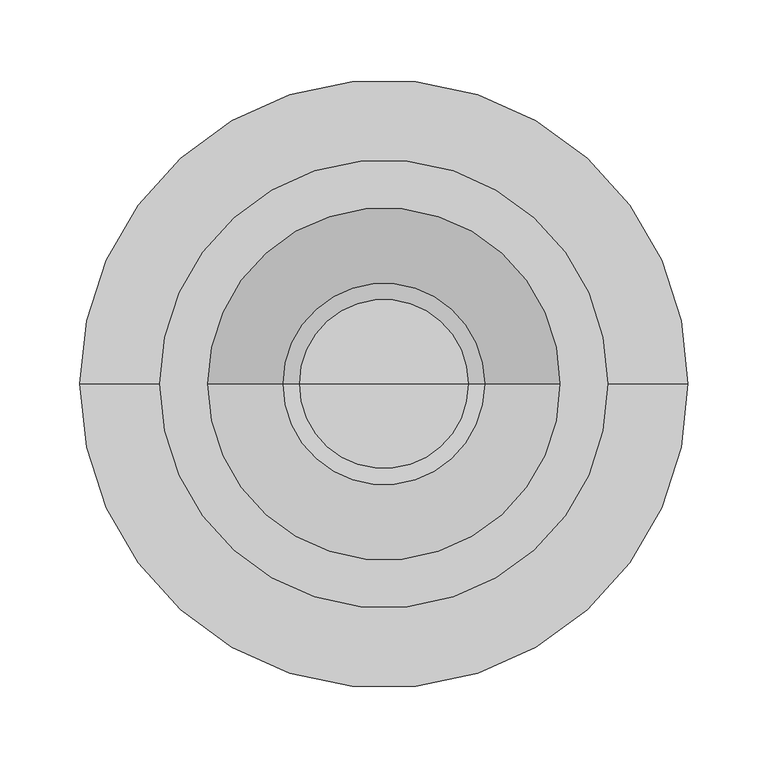
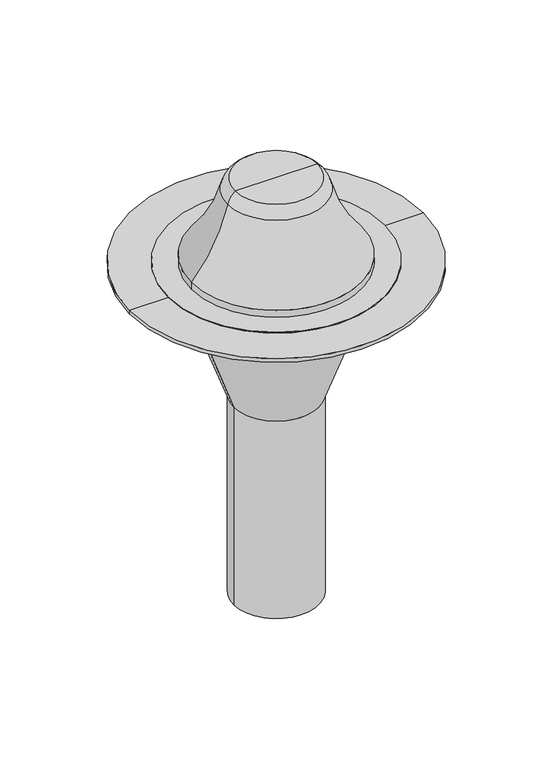
"""IFC4 building model written with IfcOpenShell, lengths in millimetres: proxy geometry, TN_Воронка с обжимным фланцем : Воронка с обжимным закручивающемся фланцем без обогрева Ø110х450мм."""

import ifcopenshell
import ifcopenshell.guid

model = None  # the IFC model being written
_history = None  # IfcOwnerHistory: only IFC2X3 demands one
_inside = {}  # id of a spatial element -> (the spatial element, [elements in it])
_under = {}  # id of a project, library or spatial element -> (it, [spatial elements below it])
_declared = {}  # id of a project -> (the project, [libraries it declares])
_typed = {}  # id of a type object -> (the type object, [elements of that type])
_made_of = {}  # id of a material, layer set ... -> (it, [elements and type objects made of it])


def new_model(schema):
    """Start an empty IFC model of exactly this schema.

    Asked for "IFC4X3", IfcOpenShell would pick the latest addendum, in which some entities
    have other attributes; the version numbers below select the first issue.
    IFC2X3 requires an IfcOwnerHistory on every rooted entity: one is made here for all.
    """
    global model, _history
    if schema == "IFC4X3":
        model = ifcopenshell.file(schema_version=(4, 3, 0, 0))
    else:
        model = ifcopenshell.file(schema=schema)
    _inside.clear()
    _under.clear()
    _declared.clear()
    _typed.clear()
    _made_of.clear()
    _history = None
    if model.schema == "IFC2X3":
        org = make("IfcOrganization", Name="unknown")
        user = make(
            "IfcPersonAndOrganization",
            ThePerson=make("IfcPerson", FamilyName="unknown"),
            TheOrganization=org,
        )
        app = make(
            "IfcApplication",
            ApplicationDeveloper=org,
            Version="unknown",
            ApplicationFullName="unknown",
            ApplicationIdentifier="unknown",
        )
        _history = make(
            "IfcOwnerHistory",
            OwningUser=user,
            OwningApplication=app,
            ChangeAction="ADDED",
            CreationDate=0,
        )
    return model


def make(cls, **values):
    """One entity of the class cls with the attributes given. An attribute that is None is left unset."""
    return model.create_entity(
        cls, **{name: value for name, value in values.items() if value is not None}
    )


def rooted(cls, **values):
    """An entity with a GlobalId (a new one), such as an element, a storey or a relation."""
    return make(cls, GlobalId=ifcopenshell.guid.new(), OwnerHistory=_history, **values)


def si_unit(unit_type, name, prefix=None):
    """IfcSIUnit, for example si_unit("LENGTHUNIT", "METRE", prefix="MILLI")."""
    return make("IfcSIUnit", UnitType=unit_type, Prefix=prefix, Name=name)


def assignment(units):
    """IfcUnitAssignment: the units of a project."""
    return None if units is None else make("IfcUnitAssignment", Units=units)


def point(xyz):
    """IfcCartesianPoint."""
    return None if xyz is None else make("IfcCartesianPoint", Coordinates=xyz)


def direction(xyz):
    """IfcDirection."""
    return None if xyz is None else make("IfcDirection", DirectionRatios=xyz)


def frame(location, z_axis=None, x_axis=None):
    """IfcAxis2Placement3D, a coordinate frame: its origin and axes. An axis left out is left unset."""
    return make(
        "IfcAxis2Placement3D",
        Location=point(location),
        Axis=direction(z_axis),
        RefDirection=direction(x_axis),
    )


def frame_2d(location, x_axis=None):
    """IfcAxis2Placement2D, a coordinate frame in the plane: its origin and x axis."""
    return make(
        "IfcAxis2Placement2D", Location=point(location), RefDirection=direction(x_axis)
    )


def origin():
    """The frame at (0, 0, 0) with its axes left unset."""
    return frame((0.0, 0.0, 0.0))


def origin_with_axes():
    """The frame at (0, 0, 0) with the z axis (0, 0, 1) and the x axis (1, 0, 0) written out."""
    return frame((0.0, 0.0, 0.0), z_axis=(0.0, 0.0, 1.0), x_axis=(1.0, 0.0, 0.0))


def origin_2d():
    """The frame at (0, 0) in the plane with its x axis left unset."""
    return frame_2d((0.0, 0.0))


def place(relative_to, where):
    """IfcLocalPlacement: puts the frame where relative to a parent placement (None: the world)."""
    return make(
        "IfcLocalPlacement", PlacementRelTo=relative_to, RelativePlacement=where
    )


def context(
    kind, dimensions, precision=None, world=None, true_north=None, identifier=None
):
    """IfcGeometricRepresentationContext, for example the 3D "Model" context."""
    return make(
        "IfcGeometricRepresentationContext",
        ContextIdentifier=identifier,
        ContextType=kind,
        CoordinateSpaceDimension=dimensions,
        Precision=precision,
        WorldCoordinateSystem=world,
        TrueNorth=true_north,
    )


def project(units=None, contexts=None):
    """IfcProject with its units and contexts."""
    return rooted(
        "IfcProject",
        Name="project",
        RepresentationContexts=contexts,
        UnitsInContext=assignment(units),
    )


def spatial(cls, under=None, at=None, **own):
    """A site, building, storey or space (cls), placed at a placement, below another one or the project."""
    s = rooted(cls, ObjectPlacement=at, **own)
    if under is not None:
        _under.setdefault(under.id(), (under, []))[1].append(s)
    return s


def polyline(points):
    """IfcPolyline through the points."""
    return make("IfcPolyline", Points=[point(p) for p in points])


def circle_curve(where, radius):
    """IfcCircle in the frame where."""
    return make("IfcCircle", Position=where, Radius=radius)


def ellipse_curve(where, semi_axis1, semi_axis2):
    """IfcEllipse in the frame where."""
    return make(
        "IfcEllipse", Position=where, SemiAxis1=semi_axis1, SemiAxis2=semi_axis2
    )


def trimmed(basis, trim1, trim2, sense, master):
    """IfcTrimmedCurve: the piece of a basis curve between two trims."""
    return make(
        "IfcTrimmedCurve",
        BasisCurve=basis,
        Trim1=trim1,
        Trim2=trim2,
        SenseAgreement=sense,
        MasterRepresentation=master,
    )


def segment(curve, same_sense, transition):
    """IfcCompositeCurveSegment."""
    return make(
        "IfcCompositeCurveSegment",
        Transition=transition,
        SameSense=same_sense,
        ParentCurve=curve,
    )


def composite_curve(segments, self_intersect=None):
    """IfcCompositeCurve: segments joined end to end."""
    return make("IfcCompositeCurve", Segments=segments, SelfIntersect=self_intersect)


def outline(outer, holes=None, kind="AREA"):
    """IfcArbitraryClosedProfileDef: a profile drawn as a closed curve; with holes, ...WithVoids."""
    if holes is None:
        return make("IfcArbitraryClosedProfileDef", ProfileType=kind, OuterCurve=outer)
    return make(
        "IfcArbitraryProfileDefWithVoids",
        ProfileType=kind,
        OuterCurve=outer,
        InnerCurves=holes,
    )


def extrude(swept, where, along, depth):
    """IfcExtrudedAreaSolid: the profile swept, set in the frame where, extruded along a direction by depth."""
    return make(
        "IfcExtrudedAreaSolid",
        SweptArea=swept,
        Position=where,
        ExtrudedDirection=direction(along),
        Depth=depth,
    )


def shape(context_of_items, identifier, shape_type, items):
    """IfcShapeRepresentation: the items that make up one representation, for example the "Body"."""
    return make(
        "IfcShapeRepresentation",
        ContextOfItems=context_of_items,
        RepresentationIdentifier=identifier,
        RepresentationType=shape_type,
        Items=items,
    )


def source(mapping_origin, context_of_items, identifier, shape_type, items):
    """IfcRepresentationMap: a shape defined once, which mapped items show again and again."""
    return make(
        "IfcRepresentationMap",
        MappingOrigin=mapping_origin,
        MappedRepresentation=shape(context_of_items, identifier, shape_type, items),
    )


def transform(
    local_origin,
    x_axis=None,
    y_axis=None,
    z_axis=None,
    scale=None,
    scale2=None,
    scale3=None,
    uniform=True,
):
    """IfcCartesianTransformationOperator3D, or its non-uniform kind. x_axis, y_axis, z_axis: its Axis1, 2, 3."""
    if uniform:
        return make(
            "IfcCartesianTransformationOperator3D",
            Axis1=direction(x_axis),
            Axis2=direction(y_axis),
            LocalOrigin=point(local_origin),
            Scale=scale,
            Axis3=direction(z_axis),
        )
    return make(
        "IfcCartesianTransformationOperator3DnonUniform",
        Axis1=direction(x_axis),
        Axis2=direction(y_axis),
        LocalOrigin=point(local_origin),
        Scale=scale,
        Axis3=direction(z_axis),
        Scale2=scale2,
        Scale3=scale3,
    )


def mapped(mapping_source, mapping_target):
    """IfcMappedItem: shows the shape of a source again, moved by a transform."""
    return make(
        "IfcMappedItem", MappingSource=mapping_source, MappingTarget=mapping_target
    )


def made_of(thing, what):
    """Note that an element or type object is made of a material, layer set ...; save() writes the relation."""
    if what is not None:
        _made_of.setdefault(what.id(), (what, []))[1].append(thing)
    return thing


def element(
    cls,
    number,
    at=None,
    inside=None,
    cuts=None,
    type_object=None,
    material=None,
    context=None,
    identifier="Body",
    shape_type=None,
    held_by="IfcProductDefinitionShape",
    body=None,
    shapes=None,
    **own,
):
    """One element of the class cls, such as IfcWall. Its Tag is "e" and its number.

    at: its placement. inside: the storey or other place that contains it. cuts: it is an
    opening in that element (IfcRelVoidsElement). A single representation is given by context,
    identifier, shape_type and body (its items); several are given by shapes. held_by: the class
    of the entity that holds the representations. save() writes the other relations.
    """
    e = rooted(cls, Tag="e%d" % number, ObjectPlacement=at, **own)
    if body is not None:
        shapes = [shape(context, identifier, shape_type, body)]
    if shapes is not None:
        e.Representation = make(held_by, Representations=shapes)
    if inside is not None:
        _inside.setdefault(inside.id(), (inside, []))[1].append(e)
    if cuts is not None:
        rooted(
            "IfcRelVoidsElement", RelatingBuildingElement=cuts, RelatedOpeningElement=e
        )
    if type_object is not None:
        _typed.setdefault(type_object.id(), (type_object, []))[1].append(e)
    return made_of(e, material)


def aggregate(whole, parts):
    """IfcRelAggregates: a whole, such as a stair, and the parts it consists of."""
    return rooted("IfcRelAggregates", RelatingObject=whole, RelatedObjects=parts)


def save(model, path):
    """Write the relations noted so far, then the file.

    IfcRelAggregates (storeys below a building ...), IfcRelContainedInSpatialStructure (elements
    in a storey), IfcRelDefinesByType, IfcRelAssociatesMaterial and IfcRelDeclares: one each for
    every whole, place, type object, material and project.
    """
    for whole, parts in _under.values():
        aggregate(whole, parts)
    for where, things in _inside.values():
        rooted(
            "IfcRelContainedInSpatialStructure",
            RelatedElements=things,
            RelatingStructure=where,
        )
    for kind, things in _typed.values():
        rooted("IfcRelDefinesByType", RelatedObjects=things, RelatingType=kind)
    for what, things in _made_of.values():
        rooted("IfcRelAssociatesMaterial", RelatedObjects=things, RelatingMaterial=what)
    for by, libraries in _declared.values():
        rooted("IfcRelDeclares", RelatingContext=by, RelatedDefinitions=libraries)
    model.write(path)


def plane_surface(at):
    """IfcPlane: the flat surface through the origin of the frame at, square to its z axis."""
    return make("IfcPlane", Position=at)


def cylinder_surface(at, radius):
    """IfcCylindricalSurface: all points at the distance radius from the z axis of the frame at."""
    return make("IfcCylindricalSurface", Position=at, Radius=radius)


def revolved_surface(curve, axis_point, axis_direction):
    """IfcSurfaceOfRevolution: the curve turned about the line through axis_point along axis_direction."""
    return make(
        "IfcSurfaceOfRevolution",
        SweptCurve=make("IfcArbitraryOpenProfileDef", ProfileType="CURVE", Curve=curve),
        AxisPosition=make("IfcAxis1Placement", Location=point(axis_point), Axis=direction(axis_direction)),
    )


def advanced_brep(points, edges, surfaces, faces):
    """IfcAdvancedBrep: a solid bounded by faces that lie on surfaces and meet in shared edges.

    An edge is (start, end): straight between two places in points (the first is 0);
    or (start, end, curve); or (start, end, curve, False) where it runs against its curve.
    A face is (place in surfaces, loops), or (place, loops, False) where it looks against
    its surface's normal. A loop lists edges by number (the first is 1), with a minus sign
    where the edge is run from its end to its start. The first loop is the outer one.
    """
    corners = [point(p) for p in points]
    vertices = [make("IfcVertexPoint", VertexGeometry=c) for c in corners]
    made = []
    for start, end, *more in edges:
        made.append(
            make(
                "IfcEdgeCurve",
                EdgeStart=vertices[start],
                EdgeEnd=vertices[end],
                EdgeGeometry=more[0] if more else make("IfcPolyline", Points=[corners[start], corners[end]]),
                SameSense=more[1] if len(more) > 1 else True,
            )
        )
    hull = []
    for where, loops, *sense in faces:
        bounds = []
        for j, loop in enumerate(loops):
            ring = [make("IfcOrientedEdge", EdgeElement=made[abs(k) - 1], Orientation=k > 0) for k in loop]
            bounds.append(
                make(
                    "IfcFaceOuterBound" if j == 0 else "IfcFaceBound",
                    Bound=make("IfcEdgeLoop", EdgeList=ring),
                    Orientation=True,
                )
            )
        hull.append(make("IfcAdvancedFace", Bounds=bounds, FaceSurface=surfaces[where], SameSense=sense[0] if sense else True))
    return make("IfcAdvancedBrep", Outer=make("IfcClosedShell", CfsFaces=hull))


def specialty_equipment_201b4a6f(model_context):
    return source(origin(), model_context, "Body", "SolidModel", [
        advanced_brep(
        [(110.0556416, 0.0, 0.0), (-110.0556416, 0.0, 0.0), (-110.0556416, 0.0, 10.0), (110.0556416, 0.0, 10.0), (0.0, 0.0, 0.0), (52.7728393, 0.0, 115.0), (-52.7728393, 0.0, 115.0), (0.0, 0.0, 115.0), (62.9807579, 0.0, 100.6532382), (-62.9807579, 0.0, 100.6532382)],
        [
            (0, 1, circle_curve(frame((0.0, 0.0, 0.0), z_axis=(0.0, 0.0, 1.0), x_axis=(-1.0, 0.0, 0.0)), 110.0556416)),
            (1, 2),
            (2, 3, circle_curve(frame((0.0, 0.0, 10.0), z_axis=(0.0, 0.0, -1.0), x_axis=(-1.0, 0.0, 0.0)), 110.0556416)),
            (3, 0),
            (1, 0, circle_curve(frame((0.0, 0.0, 0.0), z_axis=(0.0, 0.0, 1.0), x_axis=(-1.0, 0.0, 0.0)), 110.0556416)),
            (3, 2, circle_curve(frame((0.0, 0.0, 10.0), z_axis=(0.0, 0.0, -1.0), x_axis=(-1.0, 0.0, 0.0)), 110.0556416)),
            (4, 1),
            (0, 4),
            (5, 6, circle_curve(frame((0.0, 0.0, 115.0), z_axis=(0.0, 0.0, 1.0), x_axis=(-1.0, 0.0, 0.0)), 52.7728393)),
            (6, 7),
            (7, 5),
            (6, 5, circle_curve(frame((0.0, 0.0, 115.0), z_axis=(0.0, 0.0, 1.0), x_axis=(-1.0, 0.0, 0.0)), 52.7728393)),
            (8, 9, circle_curve(frame((0.0, 0.0, 100.6532382), z_axis=(0.0, 0.0, 1.0), x_axis=(-1.0, 0.0, 0.0)), 62.9807579)),
            (9, 6, circle_curve(frame((-39.8885443, 0.0, 95.0277285), z_axis=(0.0, 1.0, 0.0), x_axis=(1.0, 0.0, 0.0)), 23.7675553)),
            (5, 8, circle_curve(frame((39.8885443, 0.0, 95.0277285), z_axis=(0.0, 1.0, 0.0), x_axis=(-1.0, 0.0, 0.0)), 23.7675553)),
            (9, 8, circle_curve(frame((0.0, 0.0, 100.6532382), z_axis=(0.0, 0.0, 1.0), x_axis=(-1.0, 0.0, 0.0)), 62.9807579)),
            (2, 9, circle_curve(frame((-271.7387744, 0.0, 151.5089197), z_axis=(0.0, -1.0, 0.0), x_axis=(1.0, 0.0, 0.0)), 214.8632351)),
            (8, 3, circle_curve(frame((271.7387744, 0.0, 151.5089197), z_axis=(0.0, -1.0, 0.0), x_axis=(-1.0, 0.0, 0.0)), 214.8632351)),
        ],
        [
            cylinder_surface(frame((0.0, 0.0, 0.0), z_axis=(0.0, 0.0, -1.0), x_axis=(-1.0, 0.0, 0.0)), 110.0556416),
            plane_surface(frame((0.0, 0.0, 0.0), z_axis=(0.0, 0.0, -1.0), x_axis=(-1.0, 0.0, 0.0))),
            plane_surface(frame((0.0, 0.0, 115.0), z_axis=(0.0, 0.0, 1.0), x_axis=(-1.0, 0.0, 0.0))),
            revolved_surface(trimmed(ellipse_curve(frame((-39.8885443, 0.0, 95.0277285), z_axis=(0.0, -1.0, 0.0), x_axis=(1.0, 0.0, 0.0)), 23.7675553, 23.7675553), [point((-52.7728393, 0.0, 115.0))], [point((-62.9807579, 0.0, 100.6532382))], True, "CARTESIAN"), (0.0, 0.0, 0.0), (0.0, 0.0, -1.0)),
            revolved_surface(trimmed(ellipse_curve(frame((-271.7387744, 0.0, 151.5089197), z_axis=(0.0, 1.0, 0.0), x_axis=(1.0, 0.0, 0.0)), 214.8632351, 214.8632351), [point((-62.9807579, 0.0, 100.6532382))], [point((-110.0556416, 0.0, 10.0))], True, "CARTESIAN"), (0.0, 0.0, 0.0), (0.0, 0.0, -1.0)),
        ],
        [
            (0, [[1, 2, 3, 4]]),
            (0, [[5, -4, 6, -2]]),
            (1, [[7, -1, 8]]),
            (1, [[-8, -5, -7]]),
            (2, [[9, 10, 11]]),
            (2, [[12, -11, -10]]),
            (3, [[13, 14, -9, 15]]),
            (3, [[16, -15, -12, -14]]),
            (4, [[-3, 17, -13, 18]]),
            (4, [[-6, -18, -16, -17]]),
        ],
    ),
        extrude(outline(composite_curve([segment(trimmed(circle_curve(origin_2d(), 140.0), [point((-140.0, 0.0))], [point((140.0, 0.0))], False, "CARTESIAN"), True, "CONTINUOUS"), segment(trimmed(circle_curve(origin_2d(), 140.0), [point((140.0, 0.0))], [point((-140.0, 0.0))], False, "CARTESIAN"), True, "CONTINUOUS")], self_intersect=False), holes=[composite_curve([segment(trimmed(circle_curve(origin_2d(), 110.0556416), [point((-110.0556416, 0.0))], [point((110.0556416, 0.0))], True, "CARTESIAN"), True, "CONTINUOUS"), segment(trimmed(circle_curve(origin_2d(), 110.0556416), [point((110.0556416, 0.0))], [point((-110.0556416, 0.0))], True, "CARTESIAN"), True, "CONTINUOUS")], self_intersect=False)]), origin_with_axes(), (0.0, 0.0, 1.0), 1.0),
        advanced_brep(
        [(0.0, 0.0, -450.0), (-55.0, 0.0, -450.0), (55.0, 0.0, -450.0), (190.0, 0.0, 0.0), (-190.0, 0.0, 0.0), (-83.890873, 0.0, 0.0), (83.890873, 0.0, 0.0), (190.0, 0.0, -5.0), (-190.0, 0.0, -5.0), (93.890873, 0.0, -5.0), (-93.890873, 0.0, -5.0), (55.0, 0.0, -179.9935725), (-55.0, 0.0, -179.9935725), (-93.890873, 0.0, -71.109127), (93.890873, 0.0, -71.109127), (81.9669914, 0.0, -74.7632135), (-81.9669914, 0.0, -74.7632135), (0.0, 0.0, -74.7632135), (83.890873, 0.0, -69.3768397), (-83.890873, 0.0, -69.3768397)],
        [
            (0, 1),
            (1, 2, circle_curve(frame((0.0, 0.0, -450.0), z_axis=(0.0, 0.0, -1.0), x_axis=(-1.0, 0.0, 0.0)), 55.0)),
            (2, 0),
            (2, 1, circle_curve(frame((0.0, 0.0, -450.0), z_axis=(0.0, 0.0, -1.0), x_axis=(-1.0, 0.0, 0.0)), 55.0)),
            (3, 4, circle_curve(frame((0.0, 0.0, 0.0), z_axis=(0.0, 0.0, 1.0), x_axis=(-1.0, 0.0, 0.0)), 190.0)),
            (4, 5),
            (5, 6, circle_curve(frame((0.0, 0.0, 0.0), z_axis=(0.0, 0.0, -1.0), x_axis=(-1.0, 0.0, 0.0)), 83.890873)),
            (6, 3),
            (4, 3, circle_curve(frame((0.0, 0.0, 0.0), z_axis=(0.0, 0.0, 1.0), x_axis=(-1.0, 0.0, 0.0)), 190.0)),
            (6, 5, circle_curve(frame((0.0, 0.0, 0.0), z_axis=(0.0, 0.0, -1.0), x_axis=(-1.0, 0.0, 0.0)), 83.890873)),
            (7, 8, circle_curve(frame((0.0, 0.0, -5.0), z_axis=(0.0, 0.0, 1.0), x_axis=(-1.0, 0.0, 0.0)), 190.0)),
            (8, 4),
            (3, 7),
            (8, 7, circle_curve(frame((0.0, 0.0, -5.0), z_axis=(0.0, 0.0, 1.0), x_axis=(-1.0, 0.0, 0.0)), 190.0)),
            (9, 10, circle_curve(frame((0.0, 0.0, -5.0), z_axis=(0.0, 0.0, 1.0), x_axis=(-1.0, 0.0, 0.0)), 93.890873)),
            (10, 8),
            (7, 9),
            (10, 9, circle_curve(frame((0.0, 0.0, -5.0), z_axis=(0.0, 0.0, 1.0), x_axis=(-1.0, 0.0, 0.0)), 93.890873)),
            (11, 12, circle_curve(frame((0.0, 0.0, -179.9935725), z_axis=(0.0, 0.0, 1.0), x_axis=(-1.0, 0.0, 0.0)), 55.0)),
            (12, 13),
            (13, 14, circle_curve(frame((0.0, 0.0, -71.109127), z_axis=(0.0, 0.0, -1.0), x_axis=(-1.0, 0.0, 0.0)), 93.890873)),
            (14, 11),
            (12, 11, circle_curve(frame((0.0, 0.0, -179.9935725), z_axis=(0.0, 0.0, 1.0), x_axis=(-1.0, 0.0, 0.0)), 55.0)),
            (14, 13, circle_curve(frame((0.0, 0.0, -71.109127), z_axis=(0.0, 0.0, -1.0), x_axis=(-1.0, 0.0, 0.0)), 93.890873)),
            (1, 12),
            (11, 2),
            (15, 16, circle_curve(frame((0.0, 0.0, -74.7632135), z_axis=(0.0, 0.0, 1.0), x_axis=(-1.0, 0.0, 0.0)), 81.9669914)),
            (16, 17),
            (17, 15),
            (16, 15, circle_curve(frame((0.0, 0.0, -74.7632135), z_axis=(0.0, 0.0, 1.0), x_axis=(-1.0, 0.0, 0.0)), 81.9669914)),
            (18, 19, circle_curve(frame((0.0, 0.0, -69.3768397), z_axis=(0.0, 0.0, 1.0), x_axis=(-1.0, 0.0, 0.0)), 83.890873)),
            (19, 16),
            (15, 18),
            (19, 18, circle_curve(frame((0.0, 0.0, -69.3768397), z_axis=(0.0, 0.0, 1.0), x_axis=(-1.0, 0.0, 0.0)), 83.890873)),
            (5, 19),
            (18, 6),
            (13, 10),
            (9, 14),
        ],
        [
            plane_surface(frame((0.0, 0.0, -450.0), z_axis=(0.0, 0.0, -1.0), x_axis=(-1.0, 0.0, 0.0))),
            plane_surface(frame((0.0, 0.0, 0.0), z_axis=(0.0, 0.0, 1.0), x_axis=(-1.0, 0.0, 0.0))),
            cylinder_surface(frame((0.0, 0.0, 0.0), z_axis=(0.0, 0.0, -1.0), x_axis=(-1.0, 0.0, 0.0)), 190.0),
            plane_surface(frame((0.0, 0.0, -5.0), z_axis=(0.0, 0.0, -1.0), x_axis=(-1.0, 0.0, 0.0))),
            revolved_surface(polyline([(-93.890873, 0.0, -71.109127), (-55.0, 0.0, -179.9935725)]), (0.0, 0.0, 0.0), (0.0, 0.0, -1.0)),
            cylinder_surface(frame((0.0, 0.0, 0.0), z_axis=(0.0, 0.0, -1.0), x_axis=(-1.0, 0.0, 0.0)), 55.0),
            plane_surface(frame((0.0, 0.0, -74.7632135), z_axis=(0.0, 0.0, 1.0), x_axis=(-1.0, 0.0, 0.0))),
            revolved_surface(polyline([(-81.9669914, 0.0, -74.7632135), (-83.890873, 0.0, -69.3768397)]), (0.0, 0.0, 0.0), (0.0, 0.0, -1.0)),
            revolved_surface(polyline([(-83.890873, 0.0, -69.3768397), (-83.890873, 0.0, 0.0)]), (0.0, 0.0, 0.0), (0.0, 0.0, -1.0)),
            cylinder_surface(frame((0.0, 0.0, 0.0), z_axis=(0.0, 0.0, -1.0), x_axis=(-1.0, 0.0, 0.0)), 93.890873),
        ],
        [
            (0, [[1, 2, 3]]),
            (0, [[-3, 4, -1]]),
            (1, [[5, 6, 7, 8]]),
            (1, [[9, -8, 10, -6]]),
            (2, [[11, 12, -5, 13]]),
            (2, [[14, -13, -9, -12]]),
            (3, [[15, 16, -11, 17]]),
            (3, [[18, -17, -14, -16]]),
            (4, [[19, 20, 21, 22]]),
            (4, [[23, -22, 24, -20]]),
            (5, [[-2, 25, -19, 26]]),
            (5, [[-4, -26, -23, -25]]),
            (6, [[27, 28, 29]]),
            (6, [[30, -29, -28]]),
            (7, [[31, 32, -27, 33]]),
            (7, [[34, -33, -30, -32]]),
            (8, [[-7, 35, -31, 36]]),
            (8, [[-10, -36, -34, -35]]),
            (9, [[-21, 37, -15, 38]]),
            (9, [[-24, -38, -18, -37]]),
        ],
    ),
    ])


if __name__ == "__main__":
    model = new_model("IFC4")
    model_context = context("Model", 3, world=origin())
    ifc_project = project(units=[si_unit("LENGTHUNIT", "METRE", prefix="MILLI")], contexts=[model_context])
    site = spatial("IfcSite", under=ifc_project)
    building = spatial("IfcBuilding", under=site)
    placement = place(None, origin())
    specialty_equipment_shape = specialty_equipment_201b4a6f(model_context)
    element("IfcBuildingElementProxy", 1, Name="TN_Воронка с обжимным фланцем : Воронка с обжимным закручивающемся фланцем без обогрева Ø110х450мм", ObjectType="TN_Воронка с обжимным фланцем : Воронка с обжимным закручивающемся фланцем без обогрева Ø110х450мм", at=placement, inside=building, context=model_context, shape_type="MappedRepresentation", body=[
        mapped(specialty_equipment_shape, transform((0.0, 0.0, 0.0), x_axis=(1.0, 0.0, 0.0), y_axis=(0.0, 1.0, 0.0), z_axis=(0.0, 0.0, 1.0))),
    ])
    save(model, "model.ifc")

# Revit data of these elements
# Type "TN_Воронка с обжимным фланцем : Воронка с обжимным закручивающемся фланцем без обогрева Ø110х450мм"
#   ADSK_Группирование = "Комплектующие и воронки"
#   Description = "Кровельная воронка с обжимным закручивающимся фланцем является универсальным средством для отвода воды с поверхности плоских кровель, в устройстве которых использовались ПВХ и ТПО мембраны. Для более эффективной работы и удобства монтажа воронка оснащена обжимным закручивающимся фланцем.\r\n\r\nВоронка не оснащена обогревом и поэтому подходит для кровель неотапливаемых помещений.\r\n\r\nИспользовать воронку можно во всех климатических регионах, т.к. она не плавится при температуре до +70 С и не становится ломкой до – 55 С.\r\n\r\nДополнительно для защиты от солнца в состав добавлены УФ-стабилизаторы, обеспечивающие устойчивость к ультрафиолетовому и атмосферному воздействию в диапазоне температур от минус 50 до плюс 90 °С.\r\n\r\nБлагодаря механическому способу крепления, воронка подходит для всех типов полимерных кровельных материалов."
#   Manufacturer = "ТехноНИКОЛЬ"
#   URL = "https://shop.tn.ru/voronka-s-obzhimnym-zakruchivajuschemsja-flancem-bez-obogreva-o110h450mm#characteristics"
#   ADSK_Примечание = ""
#   ADSK_Обозначение = "ТехноНИКОЛЬ"
#   ADSK_Наименование = "Воронка с обжимным закручивающемся фланцем без обогрева Ø110х450мм"
#   ADSK_Масса_Текст = ""
#   ADSK_Марка = ""
#   ADSK_Код изделия = "661132"
#   ADSK_Завод-изготовитель = "ТехноНИКОЛЬ"
#   ADSK_Единица измерения = "шт."
#   ADSK_Группирование = "Комплектующие и воронки"
#   ADSK_URL страницы изделия = "https://shop.tn.ru/voronka-s-obzhimnym-zakruchivajuschemsja-flancem-bez-obogreva-o110h450mm#characteristics"
#   ADSK_URL документации изделия = "https://shop.tn.ru/media/other_documents/_661125_661124_661134_671701_671702_661132_661131_661130_5.pdf"
#   Тип воронки = 1
#   Радиус = 55 mm
#   Пропускная способность = 7.8 L/s
#   Монтажный диаметр = 110 mm
#   Длина расчетная [instance default] = 450 mm
#   Длина отвода [instance default] = 450 mm
#   ADSK_Масса = 2
#   ADSK_Количество = 1
#   Видимость_Листоуловитель [instance default] = yes
#   Материал_Фланец = TN_Фланец_Красный
#   Материал_Корпус = TN_ПВХ_Черный
#   Default Elevation = 0
# Element 1 (IfcBuildingElementProxy, "TN_Воронка с обжимным фланцем : Воронка с обжимным закручивающемся фланцем без обогрева Ø110х450мм")
#   Materials on its faces: "TN_ПВХ_Черный", "TN_Фланец_Красный"
# Materials
#   "TN_Фланец_Красный": class "Типовые", colour RGB 70 0 0, transparency 0, Cost = 0
#   "TN_ПВХ_Черный": class "Типовые", colour RGB 48 48 48, transparency 0, Cost = 0
